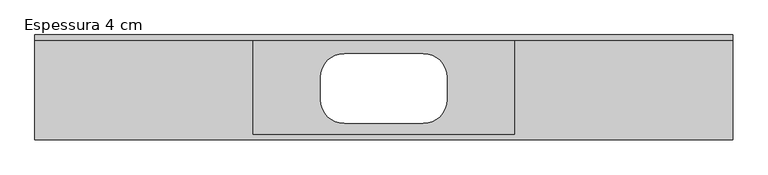
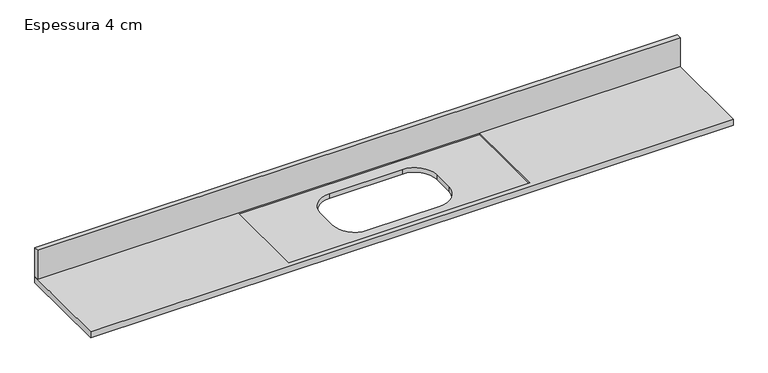
"""IFC4 building model written with IfcOpenShell, lengths in millimetres: furniture geometry, CC_BANCADA COZINHA_RETA : Espessura 4 cm."""

from ifc_helpers import new_model, si_unit, frame, origin, place, context, project, spatial, polyline, circle_curve, outline, extrude, source, transform, mapped, element, save
from ifc_brep_helpers import plane_surface, revolved_surface, advanced_brep


def espessura_4_cm_16a63bfa(model_context):
    return source(origin(), model_context, "Body", "SolidModel", [
        extrude(outline(polyline([(-4000.0, -30.0), (-4000.0, 0.0), (0.0, 0.0), (0.0, -30.0), (-4000.0, -30.0)])), frame((0.0, 0.0, 900.0), z_axis=(0.0, 0.0, 1.0), x_axis=(1.0, 0.0, 0.0)), (0.0, 0.0, 1.0), 190.0),
        advanced_brep(
        [(0.0, -600.0, 860.0), (-4000.0, -600.0, 860.0), (-4000.0, 0.0, 860.0), (0.0, 0.0, 860.0), (-2226.0, -107.0, 860.0), (-2361.0, -242.0, 860.0), (-2361.0, -372.0, 860.0), (-2226.0, -507.0, 860.0), (-1774.0, -507.0, 860.0), (-1639.0, -372.0, 860.0), (-1639.0, -242.0, 860.0), (-1774.0, -107.0, 860.0), (0.0, -600.0, 900.0), (0.0, 0.0, 900.0), (-4000.0, 0.0, 900.0), (-4000.0, -600.0, 900.0), (-1250.0, -30.0, 900.0), (-1250.0, -570.0, 900.0), (-2750.0, -570.0, 900.0), (-2750.0, -30.0, 900.0), (-1774.0, -107.0, 890.0), (-2226.0, -107.0, 890.0), (-1639.0, -242.0, 890.0), (-1639.0, -372.0, 890.0), (-1774.0, -507.0, 890.0), (-2226.0, -507.0, 890.0), (-2361.0, -372.0, 890.0), (-2361.0, -242.0, 890.0), (-1250.0, -570.0, 890.0), (-1250.0, -30.0, 890.0), (-2750.0, -30.0, 890.0), (-2750.0, -570.0, 890.0)],
        [
            (0, 1),
            (1, 2),
            (2, 3),
            (3, 0),
            (4, 5, circle_curve(frame((-2226.0, -242.0, 860.0), z_axis=(0.0, 0.0, 1.0), x_axis=(-1.0, 0.0, 0.0)), 135.0)),
            (5, 6),
            (6, 7, circle_curve(frame((-2226.0, -372.0, 860.0), z_axis=(0.0, 0.0, 1.0), x_axis=(-1.0, 0.0, 0.0)), 135.0)),
            (7, 8),
            (8, 9, circle_curve(frame((-1774.0, -372.0, 860.0), z_axis=(0.0, 0.0, 1.0), x_axis=(-1.0, 0.0, 0.0)), 135.0)),
            (9, 10),
            (10, 11, circle_curve(frame((-1774.0, -242.0, 860.0), z_axis=(0.0, 0.0, 1.0), x_axis=(-1.0, 0.0, 0.0)), 135.0)),
            (11, 4),
            (12, 13),
            (13, 14),
            (14, 15),
            (15, 12),
            (16, 17),
            (17, 18),
            (18, 19),
            (19, 16),
            (3, 13),
            (12, 0),
            (2, 14),
            (1, 15),
            (11, 20),
            (20, 21),
            (21, 4),
            (10, 22),
            (22, 20, circle_curve(frame((-1774.0, -242.0, 890.0), z_axis=(0.0, 0.0, 1.0), x_axis=(-1.0, 0.0, 0.0)), 135.0)),
            (9, 23),
            (23, 22),
            (8, 24),
            (24, 23, circle_curve(frame((-1774.0, -372.0, 890.0), z_axis=(0.0, 0.0, 1.0), x_axis=(-1.0, 0.0, 0.0)), 135.0)),
            (7, 25),
            (25, 24),
            (6, 26),
            (26, 25, circle_curve(frame((-2226.0, -372.0, 890.0), z_axis=(0.0, 0.0, 1.0), x_axis=(-1.0, 0.0, 0.0)), 135.0)),
            (5, 27),
            (27, 26),
            (21, 27, circle_curve(frame((-2226.0, -242.0, 890.0), z_axis=(0.0, 0.0, 1.0), x_axis=(-1.0, 0.0, 0.0)), 135.0)),
            (28, 29),
            (29, 30),
            (30, 31),
            (31, 28),
            (28, 17),
            (16, 29),
            (19, 30),
            (18, 31),
        ],
        [
            plane_surface(frame((0.0, -1500.0, 860.0), z_axis=(0.0, 0.0, -1.0), x_axis=(0.0, -1.0, 0.0))),
            plane_surface(frame((0.0, -1500.0, 900.0), z_axis=(0.0, 0.0, 1.0), x_axis=(0.0, 1.0, 0.0))),
            plane_surface(frame((0.0, -600.0, 900.0), z_axis=(1.0, 0.0, 0.0), x_axis=(0.0, 0.0, -1.0))),
            plane_surface(frame((0.0, 0.0, 900.0), z_axis=(0.0, 1.0, 0.0), x_axis=(0.0, 0.0, -1.0))),
            plane_surface(frame((-4000.0, 0.0, 900.0), z_axis=(-1.0, 0.0, 0.0), x_axis=(0.0, 0.0, -1.0))),
            plane_surface(frame((-4000.0, -600.0, 900.0), z_axis=(0.0, -1.0, 0.0), x_axis=(0.0, 0.0, -1.0))),
            plane_surface(frame((-2226.0, -107.0, 900.0), z_axis=(0.0, -1.0, 0.0), x_axis=(0.0, 0.0, -1.0))),
            revolved_surface(polyline([(-1909.0, -242.0, 860.0), (-1909.0, -242.0, 890.0)]), (-1774.0, -242.0, 890.0), (0.0, 0.0, -1.0)),
            plane_surface(frame((-1639.0, -242.0, 900.0), z_axis=(-1.0, 0.0, 0.0), x_axis=(0.0, 0.0, -1.0))),
            revolved_surface(polyline([(-1909.0, -372.0, 860.0), (-1909.0, -372.0, 890.0)]), (-1774.0, -372.0, 890.0), (0.0, 0.0, -1.0)),
            plane_surface(frame((-1774.0, -507.0, 900.0), z_axis=(0.0, 1.0, 0.0), x_axis=(0.0, 0.0, -1.0))),
            revolved_surface(polyline([(-2361.0, -372.0, 860.0), (-2361.0, -372.0, 890.0)]), (-2226.0, -372.0, 890.0), (0.0, 0.0, -1.0)),
            plane_surface(frame((-2361.0, -372.0, 900.0), z_axis=(1.0, 0.0, 0.0), x_axis=(0.0, 0.0, -1.0))),
            revolved_surface(polyline([(-2361.0, -242.0, 860.0), (-2361.0, -242.0, 890.0)]), (-2226.0, -242.0, 890.0), (0.0, 0.0, -1.0)),
            plane_surface(frame((-1250.0, -30.0, 890.0), z_axis=(0.0, 0.0, 1.0), x_axis=(0.0, -1.0, 0.0))),
            plane_surface(frame((-1250.0, -570.0, 940.0), z_axis=(-1.0, 0.0, 0.0), x_axis=(0.0, 0.0, -1.0))),
            plane_surface(frame((-1250.0, -30.0, 940.0), z_axis=(0.0, -1.0, 0.0), x_axis=(0.0, 0.0, -1.0))),
            plane_surface(frame((-2750.0, -30.0, 940.0), z_axis=(1.0, 0.0, 0.0), x_axis=(0.0, 0.0, -1.0))),
            plane_surface(frame((-2750.0, -570.0, 940.0), z_axis=(0.0, 1.0, 0.0), x_axis=(0.0, 0.0, -1.0))),
        ],
        [
            (0, [[1, 2, 3, 4], [5, 6, 7, 8, 9, 10, 11, 12]]),
            (1, [[13, 14, 15, 16], [17, 18, 19, 20]]),
            (2, [[-4, 21, -13, 22]]),
            (3, [[-3, 23, -14, -21]]),
            (4, [[-2, 24, -15, -23]]),
            (5, [[-1, -22, -16, -24]]),
            (6, [[-12, 25, 26, 27]]),
            (7, [[-11, 28, 29, -25]]),
            (8, [[-10, 30, 31, -28]]),
            (9, [[-9, 32, 33, -30]]),
            (10, [[-8, 34, 35, -32]]),
            (11, [[-7, 36, 37, -34]]),
            (12, [[-6, 38, 39, -36]]),
            (13, [[-5, -27, 40, -38]]),
            (14, [[41, 42, 43, 44], [-26, -29, -31, -33, -35, -37, -39, -40]]),
            (15, [[-41, 45, -17, 46]]),
            (16, [[-42, -46, -20, 47]]),
            (17, [[-43, -47, -19, 48]]),
            (18, [[-44, -48, -18, -45]]),
        ],
    ),
    ])


if __name__ == "__main__":
    model = new_model("IFC4")
    model_context = context("Model", 3, world=origin())
    ifc_project = project(units=[si_unit("LENGTHUNIT", "METRE", prefix="MILLI")], contexts=[model_context])
    site = spatial("IfcSite", under=ifc_project)
    building = spatial("IfcBuilding", under=site)
    placement = place(None, origin())
    espessura_4_cm_shape = espessura_4_cm_16a63bfa(model_context)
    element("IfcFurniture", 1, ObjectType="CC_BANCADA COZINHA_RETA : Espessura 4 cm", at=placement, inside=building, context=model_context, shape_type="MappedRepresentation", body=[
        mapped(espessura_4_cm_shape, transform((0.0, 0.0, 0.0), x_axis=(1.0, 0.0, 0.0), y_axis=(0.0, 1.0, 0.0), z_axis=(0.0, 0.0, 1.0))),
    ])
    save(model, "model.ifc")

# Revit data of these elements
# Type "CC_BANCADA COZINHA_RETA : Espessura 4 cm"
#   Uso HS [instance default] = ""
#   Offset esq área molhada [instance default] = 1.25 m
#   Largura área molhada [instance default] = 1.50 m
#   Largura principal [instance default] = 0.60 m
#   Espessura total da bancada [instance default] = 0.04 m
#   Espessura do frontão [instance default] = 0.03 m
#   Dist. cuba - borda [instance default] = 0.07 m
#   Compr. total principal [instance default] = 4.00 m
#   Altura do rebaixo da área molhada [instance default] = 0.01 m
#   Altura do frontão [instance default] = 0.20 m
#   Altura da bancada [instance default] = 0.90 m
#   Frontão fundos [instance default] = yes
#   Frontão esquerdo [instance default] = yes
#   Frontão direito [instance default] = yes
#   Material da bancada [instance default] = none
# Element 1 (IfcFurniture, "CC_BANCADA COZINHA_RETA : Espessura 4 cm")
#   Uso HS = "VARANDA"
#   Frontão esquerdo = no
#   Frontão direito = no
#   Material da bancada = .GRANITO_BRANCO_ITAUNAS
#   Materials on its faces: ".GRANITO_BRANCO_ITAUNAS"
# Materials
#   ".GRANITO_BRANCO_ITAUNAS": class ".CC_PEDRA REVEST.", colour RGB 202 195 174, transparency 0, Description = "Revestimento em granito", Cost = 0
